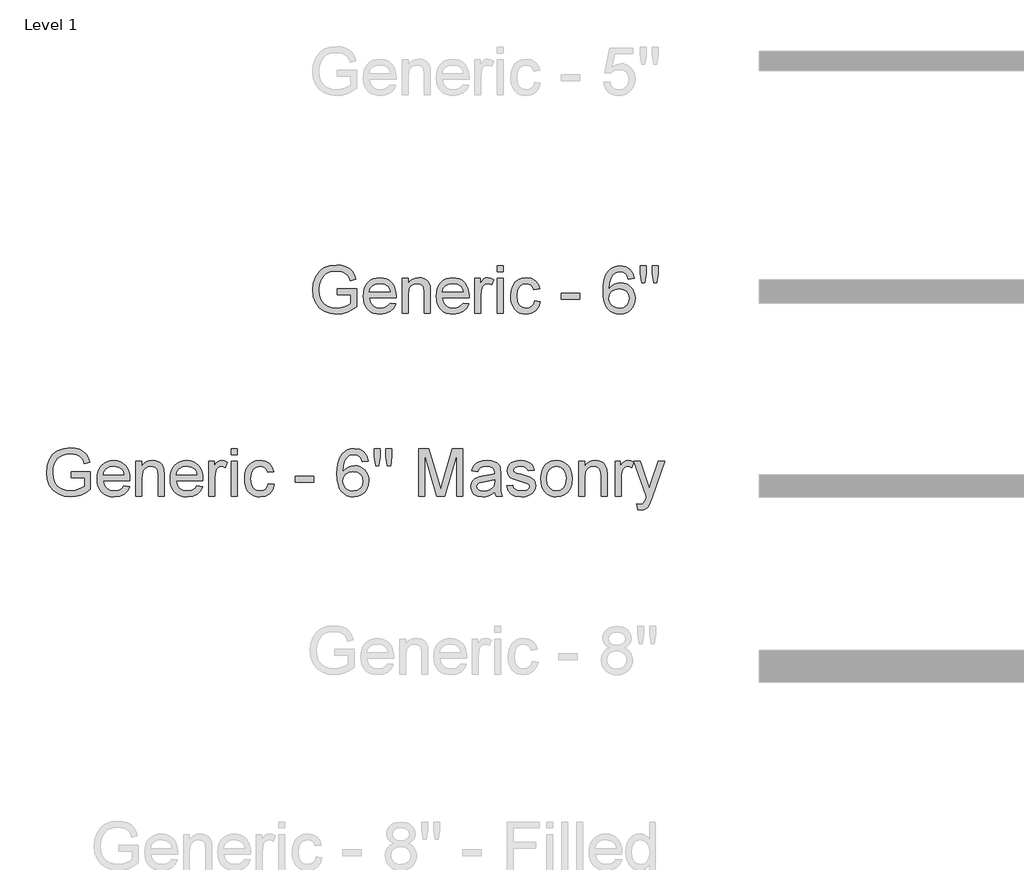
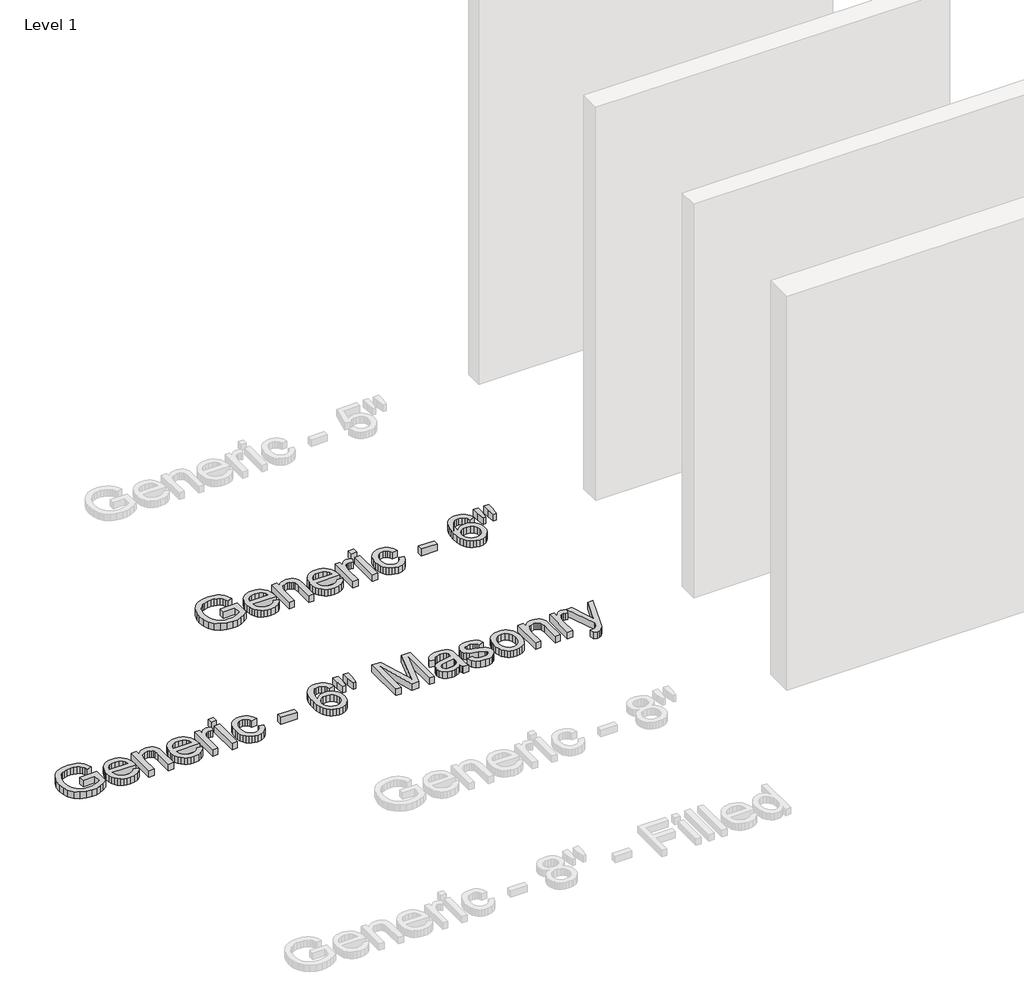
# One storey, part 24 of 42: 2 proxies.
"""IFC4 building model written with IfcOpenShell, lengths in millimetres."""

from ifc_helpers import new_model, si_unit, origin, origin_with_axes, place, context, project, spatial, polyline, outline, extrude, element, save

model = new_model("IFC4")

# Units and contexts
model_context = context("Model", 3, world=origin())
ifc_project = project(units=[si_unit("LENGTHUNIT", "METRE", prefix="MILLI")], contexts=[model_context])

# Site, building, storey
site = spatial("IfcSite", under=ifc_project)
building = spatial("IfcBuilding", under=site)
storey = spatial("IfcBuildingStorey", under=building, Name="Level 1", Elevation=0.0)

# Proxies
placement = place(None, origin())
element("IfcBuildingElementProxy", 1, Name="8\" Arial", ObjectType="8\" Arial", at=placement, inside=storey, context=model_context, shape_type="SweptSolid", body=[
    extrude(outline(polyline([(-15218.2716605, 14606.7864432), (-15218.2716605, 14644.85733), (-15094.5412786, 14644.85733), (-15094.5412786, 14531.0164557), (-15124.6094716, 14510.103493), (-15155.6257189, 14495.1019278), (-15187.5156634, 14486.0675279), (-15220.2049477, 14483.0560613), (-15262.9138649, 14487.8428061), (-15301.5145467, 14502.2030404), (-15333.5810895, 14525.6348533), (-15356.6875896, 14557.6363336), (-15370.6574487, 14596.0232384), (-15375.3140684, 14638.6113251), (-15370.676038, 14681.5061353), (-15356.7619468, 14721.4080681), (-15334.1480632, 14754.8781031), (-15319.7947998, 14767.9115262), (-15303.4106553, 14778.4772196), (-15265.9718048, 14792.4749627), (-15223.253593, 14797.140877), (-15191.8934436, 14794.4361338), (-15163.6934752, 14786.3219043), (-15139.9456442, 14773.3837514), (-15121.941907, 14756.207238), (-15108.6226734, 14733.9651404), (-15098.9283534, 14705.8302346), (-15134.0249521, 14695.9407269), (-15141.8603421, 14716.0078764), (-15151.3873585, 14731.1488614), (-15163.990904, 14742.5626917), (-15181.0558816, 14751.4483772), (-15201.4018706, 14757.164587), (-15223.8484506, 14759.0699903), (-15250.1244264, 14757.0158726), (-15272.5895956, 14750.8535196), (-15291.1603065, 14741.3543872), (-15305.7529071, 14729.2899314), (-15325.3460295, 14699.9560157), (-15334.2688936, 14671.2169576), (-15337.2431816, 14640.1728263), (-15333.6647414, 14603.7656819), (-15322.9294205, 14573.8090247), (-15305.3625318, 14550.5166316), (-15281.2893881, 14534.1022795), (-15253.1173037, 14524.3707809), (-15223.253593, 14521.126948), (-15196.8846707, 14523.571441), (-15171.1663739, 14530.9049199), (-15148.8313297, 14541.0082046), (-15132.6121653, 14551.7621147), (-15132.6121653, 14606.7864432), (-15218.2716605, 14606.7864432)])), origin_with_axes(), (0.0, 0.0, 1.0), 50.8),
    extrude(outline(polyline([(-14880.8386837, 14554.4389739), (-14843.511369, 14549.6801131), (-14856.9607277, 14521.5545019), (-14878.4220747, 14500.5300034), (-14907.4120883, 14487.4245468), (-14943.4474467, 14483.0560613), (-14967.0697999, 14484.9405516), (-14988.117535, 14490.5940225), (-15006.5906521, 14500.016474), (-15022.4891511, 14513.2079061), (-15035.2739423, 14529.8011802), (-15044.405936, 14549.4291575), (-15049.8851322, 14572.0918381), (-15051.7115309, 14597.7892219), (-15049.8665429, 14624.3579792), (-15044.3315788, 14647.7758501), (-15035.1066386, 14668.0428346), (-15022.1917223, 14685.1589328), (-15006.3350492, 14698.7570058), (-14988.2848387, 14708.4699152), (-14968.0410909, 14714.2976608), (-14945.6038055, 14716.2402427), (-14923.8891793, 14714.3023081), (-14904.2519073, 14708.4885045), (-14886.6919896, 14698.7988318), (-14871.2094262, 14685.23329), (-14858.5710258, 14668.1543704), (-14849.5435969, 14647.9245645), (-14844.1271396, 14624.5438722), (-14842.3216538, 14598.0122935), (-14842.5447254, 14587.7509998), (-15013.6406442, 14587.7509998), (-15007.0507373, 14559.2536027), (-14991.7424486, 14538.3034614), (-14969.6490653, 14525.4210764), (-14942.7038747, 14521.126948), (-14922.4415375, 14523.1160031), (-14905.37656, 14529.0831685), (-14891.508942, 14539.4002301), (-14880.8386837, 14554.4389739)]), holes=[polyline([(-15013.6406442, 14625.8218866), (-14880.3925405, 14625.8218866), (-14885.5417767, 14645.9355094), (-14895.6357667, 14660.3236277), (-14917.8313911, 14673.7079239), (-14945.7525199, 14678.1693559), (-14971.4150488, 14674.6095049), (-14992.634735, 14663.929952), (-15007.3853447, 14647.2832337), (-15013.6406442, 14625.8218866)])]), origin_with_axes(), (0.0, 0.0, 1.0), 50.8),
    extrude(outline(polyline([(-14804.250767, 14487.8149221), (-14804.250767, 14711.4813818), (-14766.1798803, 14711.4813818), (-14766.1798803, 14680.2513575), (-14752.9535932, 14695.9964948), (-14737.0690362, 14707.2430214), (-14718.5262093, 14713.9909373), (-14697.3251124, 14716.2402427), (-14678.5592139, 14714.4277859), (-14661.3734059, 14708.9904156), (-14647.0410554, 14700.6066412), (-14636.8355296, 14689.9549722), (-14625.4216993, 14661.9594861), (-14623.4140549, 14625.1526718), (-14623.4140549, 14487.8149221), (-14661.4849417, 14487.8149221), (-14661.4849417, 14620.0220249), (-14665.8720165, 14653.7058369), (-14671.941423, 14663.7347643), (-14681.3754929, 14671.5143864), (-14693.4678326, 14676.5056135), (-14707.5120489, 14678.1693559), (-14729.8099145, 14674.4329066), (-14748.8174739, 14663.2235586), (-14756.4135267, 14654.0729755), (-14761.8392787, 14641.5670238), (-14766.1798803, 14606.4890144), (-14766.1798803, 14487.8149221), (-14804.250767, 14487.8149221)])), origin_with_axes(), (0.0, 0.0, 1.0), 50.8),
    extrude(outline(polyline([(-14414.4703209, 14554.4389739), (-14377.1430062, 14549.6801131), (-14390.5923649, 14521.5545019), (-14412.0537119, 14500.5300034), (-14441.0437255, 14487.4245468), (-14477.0790839, 14483.0560613), (-14500.7014371, 14484.9405516), (-14521.7491723, 14490.5940225), (-14540.2222893, 14500.016474), (-14556.1207883, 14513.2079061), (-14568.9055795, 14529.8011802), (-14578.0375732, 14549.4291575), (-14583.5167694, 14572.0918381), (-14585.3431682, 14597.7892219), (-14583.4981801, 14624.3579792), (-14577.963216, 14647.7758501), (-14568.7382758, 14668.0428346), (-14555.8233595, 14685.1589328), (-14539.9666864, 14698.7570058), (-14521.916476, 14708.4699152), (-14501.6727281, 14714.2976608), (-14479.2354428, 14716.2402427), (-14457.5208165, 14714.3023081), (-14437.8835445, 14708.4885045), (-14420.3236268, 14698.7988318), (-14404.8410635, 14685.23329), (-14392.202663, 14668.1543704), (-14383.1752341, 14647.9245645), (-14377.7587768, 14624.5438722), (-14375.953291, 14598.0122935), (-14376.1763626, 14587.7509998), (-14547.2722814, 14587.7509998), (-14540.6823745, 14559.2536027), (-14525.3740858, 14538.3034614), (-14503.2807025, 14525.4210764), (-14476.3355119, 14521.126948), (-14456.0731747, 14523.1160031), (-14439.0081972, 14529.0831685), (-14425.1405792, 14539.4002301), (-14414.4703209, 14554.4389739)]), holes=[polyline([(-14547.2722814, 14625.8218866), (-14414.0241777, 14625.8218866), (-14419.1734139, 14645.9355094), (-14429.2674039, 14660.3236277), (-14451.4630283, 14673.7079239), (-14479.3841572, 14678.1693559), (-14505.046686, 14674.6095049), (-14526.2663722, 14663.929952), (-14541.0169819, 14647.2832337), (-14547.2722814, 14625.8218866)])]), origin_with_axes(), (0.0, 0.0, 1.0), 50.8),
    extrude(outline(polyline([(-14337.8824042, 14487.8149221), (-14337.8824042, 14711.4813818), (-14304.5703783, 14711.4813818), (-14304.5703783, 14678.3924275), (-14292.2642616, 14697.5765853), (-14280.9247885, 14708.8788798), (-14269.5481368, 14714.3999019), (-14257.1304843, 14716.2402427), (-14238.1693981, 14713.3031332), (-14218.9108831, 14704.4918049), (-14231.6259644, 14670.3618498), (-14245.0102605, 14676.2174794), (-14258.3945567, 14678.1693559), (-14269.7619137, 14676.2918366), (-14279.9209663, 14670.6592786), (-14288.1281423, 14661.6992359), (-14293.6398698, 14649.8392624), (-14298.2686056, 14628.573103), (-14299.8115175, 14605.3736564), (-14299.8115175, 14487.8149221), (-14337.8824042, 14487.8149221)])), origin_with_axes(), (0.0, 0.0, 1.0), 50.8),
    extrude(outline(polyline([(-14195.1165789, 14754.3111294), (-14195.1165789, 14792.3820162), (-14157.0456921, 14792.3820162), (-14157.0456921, 14754.3111294), (-14195.1165789, 14754.3111294)])), origin_with_axes(), (0.0, 0.0, 1.0), 50.8),
    extrude(outline(polyline([(-14195.1165789, 14487.8149221), (-14195.1165789, 14711.4813818), (-14157.0456921, 14711.4813818), (-14157.0456921, 14487.8149221), (-14195.1165789, 14487.8149221)])), origin_with_axes(), (0.0, 0.0, 1.0), 50.8),
    extrude(outline(polyline([(-13957.1735366, 14568.7155565), (-13919.1026499, 14563.9566956), (-13929.7171403, 14530.0962853), (-13949.6634594, 14504.5081137), (-13977.0640878, 14488.4190744), (-14010.0415063, 14483.0560613), (-14031.3936413, 14484.9266096), (-14050.5382968, 14490.5382546), (-14067.4754729, 14499.8909962), (-14082.2051696, 14512.9848345), (-14094.127882, 14529.5734613), (-14102.6441052, 14549.4105682), (-14107.753839, 14572.4961554), (-14109.4570837, 14598.8302227), (-14106.5478582, 14632.7092223), (-14097.8201818, 14662.0710219), (-14083.1346346, 14685.7816743), (-14062.351797, 14702.7072321), (-14037.488608, 14712.85699), (-14010.5620067, 14716.2402427), (-13978.3932228, 14711.5929176), (-13952.674926, 14697.6509425), (-13934.2250456, 14675.1578893), (-13923.8615107, 14644.85733), (-13961.9323975, 14640.0984691), (-13968.8383225, 14656.7080088), (-13979.5922327, 14668.6144556), (-13993.5992703, 14675.7806308), (-14010.2645779, 14678.1693559), (-14034.8675167, 14673.4662629), (-14054.3955766, 14659.3569841), (-14067.1385418, 14635.0793581), (-14071.3861969, 14599.8712236), (-14067.2314883, 14564.1890619), (-14054.7673626, 14539.827784), (-14035.5924994, 14525.802157), (-14011.3055787, 14521.126948), (-13991.5916259, 14524.0454681), (-13975.4282294, 14532.8010285), (-13963.6704971, 14547.6167008), (-13957.1735366, 14568.7155565)])), origin_with_axes(), (0.0, 0.0, 1.0), 50.8),
    extrude(outline(polyline([(-13785.8545462, 14578.2332782), (-13785.8545462, 14616.3041649), (-13666.8830251, 14616.3041649), (-13666.8830251, 14578.2332782), (-13785.8545462, 14578.2332782)])), origin_with_axes(), (0.0, 0.0, 1.0), 50.8),
    extrude(outline(polyline([(-13319.4861834, 14711.4813818), (-13357.5570702, 14706.722521), (-13363.6915392, 14725.5906606), (-13371.9823671, 14738.4730457), (-13389.251827, 14750.3516085), (-13410.1276111, 14754.3111294), (-13427.8246249, 14752.0060562), (-13444.4806378, 14745.0908365), (-13458.7851043, 14730.5261198), (-13470.4684795, 14710.4775596), (-13478.3596374, 14682.1195822), (-13481.2874522, 14642.626614), (-13466.0163421, 14660.4444582), (-13447.715176, 14673.0015304), (-13427.4063656, 14680.4465452), (-13406.1123222, 14682.9282167), (-13387.8204509, 14681.2319431), (-13370.9413663, 14676.1431222), (-13355.4750686, 14667.661754), (-13341.4215576, 14655.7878385), (-13329.7428298, 14641.2277691), (-13321.4008814, 14624.6879393), (-13316.3957123, 14606.168349), (-13314.7273226, 14585.6689982), (-13317.8689143, 14558.4077895), (-13327.2936895, 14533.1356359), (-13342.2208975, 14511.7021728), (-13361.8697878, 14495.9570356), (-13385.348074, 14486.2813048), (-13411.7634695, 14483.0560613), (-13434.4586814, 14485.1938308), (-13454.9557085, 14491.6071393), (-13473.2545508, 14502.2959869), (-13489.3552084, 14517.2603736), (-13502.481578, 14537.1323355), (-13511.8575563, 14562.5439088), (-13517.4831433, 14593.4950936), (-13519.3583389, 14629.9858898), (-13517.2763373, 14670.8962922), (-13511.0303324, 14705.8116453), (-13500.6203243, 14734.731949), (-13486.046313, 14757.6572034), (-13470.2500552, 14772.849309), (-13451.9349472, 14783.700813), (-13431.100989, 14790.2117154), (-13407.7481807, 14792.3820162), (-13374.3432082, 14787.0097084), (-13347.5932053, 14770.8927852), (-13328.8551907, 14745.2953188), (-13319.4861834, 14711.4813818)]), holes=[polyline([(-13481.2874522, 14586.2638558), (-13479.0846201, 14569.3940659), (-13472.4761239, 14553.2864373), (-13462.2148302, 14539.4374087), (-13449.0536057, 14529.3434187), (-13433.1690487, 14523.1810657), (-13414.7377575, 14521.126948), (-13389.6143183, 14525.3838978), (-13369.8631869, 14538.154747), (-13357.0644537, 14558.2311912), (-13352.7982093, 14584.4049258), (-13357.0086858, 14609.528365), (-13369.6401153, 14628.6846388), (-13389.7258541, 14640.8141572), (-13416.2992587, 14644.85733), (-13441.3855193, 14640.8141572), (-13462.3635446, 14628.6846388), (-13476.5564753, 14609.9930975), (-13481.2874522, 14586.2638558)])]), origin_with_axes(), (0.0, 0.0, 1.0), 50.8),
    extrude(outline(polyline([(-13272.1206466, 14682.9282167), (-13281.4152967, 14741.7447625), (-13281.4152967, 14792.3820162), (-13243.3444099, 14792.3820162), (-13243.3444099, 14741.7447625), (-13251.6724164, 14682.9282167), (-13272.1206466, 14682.9282167)])), origin_with_axes(), (0.0, 0.0, 1.0), 50.8),
    extrude(outline(polyline([(-13196.2019447, 14682.9282167), (-13205.2735232, 14741.7447625), (-13205.2735232, 14792.3820162), (-13167.2026364, 14792.3820162), (-13167.2026364, 14741.7447625), (-13176.1255005, 14682.9282167), (-13196.2019447, 14682.9282167)])), origin_with_axes(), (0.0, 0.0, 1.0), 50.8),
])
element("IfcBuildingElementProxy", 2, Name="8\" Arial", ObjectType="8\" Arial", at=placement, inside=storey, context=model_context, shape_type="SweptSolid", body=[
    extrude(outline(polyline([(-16920.0716605, 13438.3864432), (-16920.0716605, 13476.45733), (-16796.3412786, 13476.45733), (-16796.3412786, 13362.6164557), (-16826.4094716, 13341.703493), (-16857.4257189, 13326.7019278), (-16889.3156634, 13317.6675279), (-16922.0049477, 13314.6560613), (-16964.7138649, 13319.4428061), (-17003.3145467, 13333.8030404), (-17035.3810895, 13357.2348533), (-17058.4875896, 13389.2363336), (-17072.4574487, 13427.6232384), (-17077.1140684, 13470.2113251), (-17072.476038, 13513.1061353), (-17058.5619468, 13553.0080681), (-17035.9480632, 13586.4781031), (-17021.5947998, 13599.5115262), (-17005.2106553, 13610.0772196), (-16967.7718048, 13624.0749627), (-16925.053593, 13628.740877), (-16893.6934436, 13626.0361338), (-16865.4934752, 13617.9219043), (-16841.7456442, 13604.9837514), (-16823.741907, 13587.807238), (-16810.4226734, 13565.5651404), (-16800.7283534, 13537.4302346), (-16835.8249521, 13527.5407269), (-16843.6603421, 13547.6078764), (-16853.1873585, 13562.7488614), (-16865.790904, 13574.1626917), (-16882.8558816, 13583.0483772), (-16903.2018706, 13588.764587), (-16925.6484506, 13590.6699903), (-16951.9244264, 13588.6158726), (-16974.3895956, 13582.4535196), (-16992.9603065, 13572.9543872), (-17007.5529071, 13560.8899314), (-17027.1460295, 13531.5560157), (-17036.0688936, 13502.8169576), (-17039.0431816, 13471.7728263), (-17035.4647414, 13435.3656819), (-17024.7294205, 13405.4090247), (-17007.1625318, 13382.1166316), (-16983.0893881, 13365.7022795), (-16954.9173037, 13355.9707809), (-16925.053593, 13352.726948), (-16898.6846707, 13355.171441), (-16872.9663739, 13362.5049199), (-16850.6313297, 13372.6082046), (-16834.4121653, 13383.3621147), (-16834.4121653, 13438.3864432), (-16920.0716605, 13438.3864432)])), origin_with_axes(), (0.0, 0.0, 1.0), 50.8),
    extrude(outline(polyline([(-16582.6386837, 13386.0389739), (-16545.311369, 13381.2801131), (-16558.7607277, 13353.1545019), (-16580.2220747, 13332.1300034), (-16609.2120883, 13319.0245468), (-16645.2474467, 13314.6560613), (-16668.8697999, 13316.5405516), (-16689.917535, 13322.1940225), (-16708.3906521, 13331.616474), (-16724.2891511, 13344.8079061), (-16737.0739423, 13361.4011802), (-16746.205936, 13381.0291575), (-16751.6851322, 13403.6918381), (-16753.5115309, 13429.3892219), (-16751.6665429, 13455.9579792), (-16746.1315788, 13479.3758501), (-16736.9066386, 13499.6428346), (-16723.9917223, 13516.7589328), (-16708.1350492, 13530.3570058), (-16690.0848387, 13540.0699152), (-16669.8410909, 13545.8976608), (-16647.4038055, 13547.8402427), (-16625.6891793, 13545.9023081), (-16606.0519073, 13540.0885045), (-16588.4919896, 13530.3988318), (-16573.0094262, 13516.83329), (-16560.3710258, 13499.7543704), (-16551.3435969, 13479.5245645), (-16545.9271396, 13456.1438722), (-16544.1216538, 13429.6122935), (-16544.3447254, 13419.3509998), (-16715.4406442, 13419.3509998), (-16708.8507373, 13390.8536027), (-16693.5424486, 13369.9034614), (-16671.4490653, 13357.0210764), (-16644.5038747, 13352.726948), (-16624.2415375, 13354.7160031), (-16607.17656, 13360.6831685), (-16593.308942, 13371.0002301), (-16582.6386837, 13386.0389739)]), holes=[polyline([(-16715.4406442, 13457.4218866), (-16582.1925405, 13457.4218866), (-16587.3417767, 13477.5355094), (-16597.4357667, 13491.9236277), (-16619.6313911, 13505.3079239), (-16647.5525199, 13509.7693559), (-16673.2150488, 13506.2095049), (-16694.434735, 13495.529952), (-16709.1853447, 13478.8832337), (-16715.4406442, 13457.4218866)])]), origin_with_axes(), (0.0, 0.0, 1.0), 50.8),
    extrude(outline(polyline([(-16506.050767, 13319.4149221), (-16506.050767, 13543.0813818), (-16467.9798803, 13543.0813818), (-16467.9798803, 13511.8513575), (-16454.7535932, 13527.5964948), (-16438.8690362, 13538.8430214), (-16420.3262093, 13545.5909373), (-16399.1251124, 13547.8402427), (-16380.3592139, 13546.0277859), (-16363.1734059, 13540.5904156), (-16348.8410554, 13532.2066412), (-16338.6355296, 13521.5549722), (-16327.2216993, 13493.5594861), (-16325.2140549, 13456.7526718), (-16325.2140549, 13319.4149221), (-16363.2849417, 13319.4149221), (-16363.2849417, 13451.6220249), (-16367.6720165, 13485.3058369), (-16373.741423, 13495.3347643), (-16383.1754929, 13503.1143864), (-16395.2678326, 13508.1056135), (-16409.3120489, 13509.7693559), (-16431.6099145, 13506.0329066), (-16450.6174739, 13494.8235586), (-16458.2135267, 13485.6729755), (-16463.6392787, 13473.1670238), (-16467.9798803, 13438.0890144), (-16467.9798803, 13319.4149221), (-16506.050767, 13319.4149221)])), origin_with_axes(), (0.0, 0.0, 1.0), 50.8),
    extrude(outline(polyline([(-16116.2703209, 13386.0389739), (-16078.9430062, 13381.2801131), (-16092.3923649, 13353.1545019), (-16113.8537119, 13332.1300034), (-16142.8437255, 13319.0245468), (-16178.8790839, 13314.6560613), (-16202.5014371, 13316.5405516), (-16223.5491723, 13322.1940225), (-16242.0222893, 13331.616474), (-16257.9207883, 13344.8079061), (-16270.7055795, 13361.4011802), (-16279.8375732, 13381.0291575), (-16285.3167694, 13403.6918381), (-16287.1431682, 13429.3892219), (-16285.2981801, 13455.9579792), (-16279.763216, 13479.3758501), (-16270.5382758, 13499.6428346), (-16257.6233595, 13516.7589328), (-16241.7666864, 13530.3570058), (-16223.716476, 13540.0699152), (-16203.4727281, 13545.8976608), (-16181.0354428, 13547.8402427), (-16159.3208165, 13545.9023081), (-16139.6835445, 13540.0885045), (-16122.1236268, 13530.3988318), (-16106.6410635, 13516.83329), (-16094.002663, 13499.7543704), (-16084.9752341, 13479.5245645), (-16079.5587768, 13456.1438722), (-16077.753291, 13429.6122935), (-16077.9763626, 13419.3509998), (-16249.0722814, 13419.3509998), (-16242.4823745, 13390.8536027), (-16227.1740858, 13369.9034614), (-16205.0807025, 13357.0210764), (-16178.1355119, 13352.726948), (-16157.8731747, 13354.7160031), (-16140.8081972, 13360.6831685), (-16126.9405792, 13371.0002301), (-16116.2703209, 13386.0389739)]), holes=[polyline([(-16249.0722814, 13457.4218866), (-16115.8241777, 13457.4218866), (-16120.9734139, 13477.5355094), (-16131.0674039, 13491.9236277), (-16153.2630283, 13505.3079239), (-16181.1841572, 13509.7693559), (-16206.846686, 13506.2095049), (-16228.0663722, 13495.529952), (-16242.8169819, 13478.8832337), (-16249.0722814, 13457.4218866)])]), origin_with_axes(), (0.0, 0.0, 1.0), 50.8),
    extrude(outline(polyline([(-16039.6824042, 13319.4149221), (-16039.6824042, 13543.0813818), (-16006.3703783, 13543.0813818), (-16006.3703783, 13509.9924275), (-15994.0642616, 13529.1765853), (-15982.7247885, 13540.4788798), (-15971.3481368, 13545.9999019), (-15958.9304843, 13547.8402427), (-15939.9693981, 13544.9031332), (-15920.7108831, 13536.0918049), (-15933.4259644, 13501.9618498), (-15946.8102605, 13507.8174794), (-15960.1945567, 13509.7693559), (-15971.5619137, 13507.8918366), (-15981.7209663, 13502.2592786), (-15989.9281423, 13493.2992359), (-15995.4398698, 13481.4392624), (-16000.0686056, 13460.173103), (-16001.6115175, 13436.9736564), (-16001.6115175, 13319.4149221), (-16039.6824042, 13319.4149221)])), origin_with_axes(), (0.0, 0.0, 1.0), 50.8),
    extrude(outline(polyline([(-15896.9165789, 13585.9111294), (-15896.9165789, 13623.9820162), (-15858.8456921, 13623.9820162), (-15858.8456921, 13585.9111294), (-15896.9165789, 13585.9111294)])), origin_with_axes(), (0.0, 0.0, 1.0), 50.8),
    extrude(outline(polyline([(-15896.9165789, 13319.4149221), (-15896.9165789, 13543.0813818), (-15858.8456921, 13543.0813818), (-15858.8456921, 13319.4149221), (-15896.9165789, 13319.4149221)])), origin_with_axes(), (0.0, 0.0, 1.0), 50.8),
    extrude(outline(polyline([(-15658.9735366, 13400.3155565), (-15620.9026499, 13395.5566956), (-15631.5171403, 13361.6962853), (-15651.4634594, 13336.1081137), (-15678.8640878, 13320.0190744), (-15711.8415063, 13314.6560613), (-15733.1936413, 13316.5266096), (-15752.3382968, 13322.1382546), (-15769.2754729, 13331.4909962), (-15784.0051696, 13344.5848345), (-15795.927882, 13361.1734613), (-15804.4441052, 13381.0105682), (-15809.553839, 13404.0961554), (-15811.2570837, 13430.4302227), (-15808.3478582, 13464.3092223), (-15799.6201818, 13493.6710219), (-15784.9346346, 13517.3816743), (-15764.151797, 13534.3072321), (-15739.288608, 13544.45699), (-15712.3620067, 13547.8402427), (-15680.1932228, 13543.1929176), (-15654.474926, 13529.2509425), (-15636.0250456, 13506.7578893), (-15625.6615107, 13476.45733), (-15663.7323975, 13471.6984691), (-15670.6383225, 13488.3080088), (-15681.3922327, 13500.2144556), (-15695.3992703, 13507.3806308), (-15712.0645779, 13509.7693559), (-15736.6675167, 13505.0662629), (-15756.1955766, 13490.9569841), (-15768.9385418, 13466.6793581), (-15773.1861969, 13431.4712236), (-15769.0314883, 13395.7890619), (-15756.5673626, 13371.427784), (-15737.3924994, 13357.402157), (-15713.1055787, 13352.726948), (-15693.3916259, 13355.6454681), (-15677.2282294, 13364.4010285), (-15665.4704971, 13379.2167008), (-15658.9735366, 13400.3155565)])), origin_with_axes(), (0.0, 0.0, 1.0), 50.8),
    extrude(outline(polyline([(-15487.6545462, 13409.8332782), (-15487.6545462, 13447.9041649), (-15368.6830251, 13447.9041649), (-15368.6830251, 13409.8332782), (-15487.6545462, 13409.8332782)])), origin_with_axes(), (0.0, 0.0, 1.0), 50.8),
    extrude(outline(polyline([(-15021.2861834, 13543.0813818), (-15059.3570702, 13538.322521), (-15065.4915392, 13557.1906606), (-15073.7823671, 13570.0730457), (-15091.051827, 13581.9516085), (-15111.9276111, 13585.9111294), (-15129.6246249, 13583.6060562), (-15146.2806378, 13576.6908365), (-15160.5851043, 13562.1261198), (-15172.2684795, 13542.0775596), (-15180.1596374, 13513.7195822), (-15183.0874522, 13474.226614), (-15167.8163421, 13492.0444582), (-15149.515176, 13504.6015304), (-15129.2063656, 13512.0465452), (-15107.9123222, 13514.5282167), (-15089.6204509, 13512.8319431), (-15072.7413663, 13507.7431222), (-15057.2750686, 13499.261754), (-15043.2215576, 13487.3878385), (-15031.5428298, 13472.8277691), (-15023.2008814, 13456.2879393), (-15018.1957123, 13437.768349), (-15016.5273226, 13417.2689982), (-15019.6689143, 13390.0077895), (-15029.0936895, 13364.7356359), (-15044.0208975, 13343.3021728), (-15063.6697878, 13327.5570356), (-15087.148074, 13317.8813048), (-15113.5634695, 13314.6560613), (-15136.2586814, 13316.7938308), (-15156.7557085, 13323.2071393), (-15175.0545508, 13333.8959869), (-15191.1552084, 13348.8603736), (-15204.281578, 13368.7323355), (-15213.6575563, 13394.1439088), (-15219.2831433, 13425.0950936), (-15221.1583389, 13461.5858898), (-15219.0763373, 13502.4962922), (-15212.8303324, 13537.4116453), (-15202.4203243, 13566.331949), (-15187.846313, 13589.2572034), (-15172.0500552, 13604.449309), (-15153.7349472, 13615.300813), (-15132.900989, 13621.8117154), (-15109.5481807, 13623.9820162), (-15076.1432082, 13618.6097084), (-15049.3932053, 13602.4927852), (-15030.6551907, 13576.8953188), (-15021.2861834, 13543.0813818)]), holes=[polyline([(-15183.0874522, 13417.8638558), (-15180.8846201, 13400.9940659), (-15174.2761239, 13384.8864373), (-15164.0148302, 13371.0374087), (-15150.8536057, 13360.9434187), (-15134.9690487, 13354.7810657), (-15116.5377575, 13352.726948), (-15091.4143183, 13356.9838978), (-15071.6631869, 13369.754747), (-15058.8644537, 13389.8311912), (-15054.5982093, 13416.0049258), (-15058.8086858, 13441.128365), (-15071.4401153, 13460.2846388), (-15091.5258541, 13472.4141572), (-15118.0992587, 13476.45733), (-15143.1855193, 13472.4141572), (-15164.1635446, 13460.2846388), (-15178.3564753, 13441.5930975), (-15183.0874522, 13417.8638558)])]), origin_with_axes(), (0.0, 0.0, 1.0), 50.8),
    extrude(outline(polyline([(-14973.9206466, 13514.5282167), (-14983.2152967, 13573.3447625), (-14983.2152967, 13623.9820162), (-14945.1444099, 13623.9820162), (-14945.1444099, 13573.3447625), (-14953.4724164, 13514.5282167), (-14973.9206466, 13514.5282167)])), origin_with_axes(), (0.0, 0.0, 1.0), 50.8),
    extrude(outline(polyline([(-14898.0019447, 13514.5282167), (-14907.0735232, 13573.3447625), (-14907.0735232, 13623.9820162), (-14869.0026364, 13623.9820162), (-14869.0026364, 13573.3447625), (-14877.9255005, 13514.5282167), (-14898.0019447, 13514.5282167)])), origin_with_axes(), (0.0, 0.0, 1.0), 50.8),
    extrude(outline(polyline([(-14697.683646, 13319.4149221), (-14697.683646, 13623.9820162), (-14632.1749522, 13623.9820162), (-14569.863618, 13409.3127777), (-14557.2972511, 13364.4753857), (-14543.6898833, 13413.0306378), (-14482.41955, 13623.9820162), (-14416.9108561, 13623.9820162), (-14416.9108561, 13319.4149221), (-14454.9817429, 13319.4149221), (-14454.9817429, 13585.9111294), (-14531.4953024, 13319.4149221), (-14583.0991997, 13319.4149221), (-14659.6127592, 13585.9111294), (-14659.6127592, 13319.4149221), (-14697.683646, 13319.4149221)])), origin_with_axes(), (0.0, 0.0, 1.0), 50.8),
    extrude(outline(polyline([(-14212.2798398, 13347.9680872), (-14230.46947, 13332.3716643), (-14249.19819, 13322.1661385), (-14268.8935535, 13316.5335806), (-14289.9831145, 13314.6560613), (-14321.7987018, 13319.1732612), (-14345.2676933, 13332.724861), (-14359.7394635, 13353.3032163), (-14364.5633868, 13378.9006827), (-14362.7416354, 13394.6829985), (-14357.2763812, 13409.0153489), (-14348.8461336, 13421.2842871), (-14338.129402, 13430.876366), (-14311.4723455, 13443.3683757), (-14278.5321056, 13449.0938801), (-14239.6061111, 13455.1168134), (-14212.5029114, 13462.1807474), (-14212.2798398, 13470.6574683), (-14214.9009311, 13487.6480887), (-14222.7642051, 13498.7644902), (-14240.3496831, 13507.0181395), (-14264.8503807, 13509.7693559), (-14287.5293269, 13507.9383098), (-14303.3674107, 13502.4451716), (-14314.1677941, 13492.2861191), (-14321.7336392, 13476.45733), (-14359.804526, 13481.2161908), (-14353.1960298, 13502.036207), (-14343.334406, 13518.3947912), (-14329.2994844, 13530.9053902), (-14310.1710945, 13540.181451), (-14286.7764603, 13545.9255447), (-14259.9428055, 13547.8402427), (-14234.2059194, 13546.1486163), (-14213.8041624, 13541.0737374), (-14198.4215165, 13533.4428297), (-14187.7419636, 13524.083117), (-14180.6594402, 13512.5112777), (-14176.0678831, 13498.2439898), (-14174.2089531, 13464.9319639), (-14174.2089531, 13417.566427), (-14172.2756658, 13351.425697), (-14164.6912314, 13319.4149221), (-14202.7621181, 13319.4149221), (-14208.8594086, 13332.6505038), (-14212.2798398, 13347.9680872)]), holes=[polyline([(-14212.2798398, 13424.1098607), (-14273.6988876, 13412.4357802), (-14306.4532345, 13406.2641325), (-14321.287496, 13396.2259104), (-14326.4925001, 13381.5775419), (-14323.6576318, 13370.2566581), (-14315.153027, 13360.9805973), (-14301.1645786, 13354.7903603), (-14281.8781797, 13352.726948), (-14261.4299495, 13355.0041373), (-14243.3611497, 13361.8357051), (-14228.7127812, 13371.9018111), (-14218.5258447, 13383.8826151), (-14214.0086447, 13396.2259104), (-14212.5029114, 13413.3280666), (-14212.2798398, 13424.1098607)])]), origin_with_axes(), (0.0, 0.0, 1.0), 50.8),
    extrude(outline(polyline([(-14136.1380663, 13386.0389739), (-14098.0671795, 13390.7978348), (-14092.0628356, 13374.5136078), (-14080.444523, 13362.5420985), (-14063.1378845, 13355.1807356), (-14040.068563, 13352.726948), (-14017.278081, 13354.9762533), (-14001.2541042, 13361.7241693), (-13991.7735611, 13371.5021412), (-13988.6133801, 13382.8416143), (-13991.7921504, 13392.545229), (-14001.3284614, 13399.9437705), (-14040.5147062, 13410.7999218), (-14097.8441079, 13429.4264005), (-14112.3530567, 13438.7861132), (-14122.865306, 13451.1758817), (-14129.2507306, 13465.805661), (-14131.3792055, 13481.8854056), (-14129.6689898, 13496.6360153), (-14124.538343, 13510.2526777), (-14116.4519974, 13522.1963031), (-14105.8746856, 13531.9278017), (-14081.6714168, 13543.1929176), (-14048.9170699, 13547.8402427), (-14024.1375327, 13545.972018), (-14002.5925338, 13540.367344), (-13985.2673061, 13531.574605), (-13973.1470824, 13520.1421854), (-13965.1165047, 13505.224272), (-13960.060215, 13485.9750517), (-13998.1311018, 13481.2161908), (-14002.9364359, 13493.1969948), (-14012.4448629, 13502.2221), (-14026.7493294, 13507.8825419), (-14045.9427818, 13509.7693559), (-14067.8037989, 13507.9661938), (-14082.3778102, 13502.5567074), (-14090.5756916, 13494.7492014), (-14093.3083187, 13485.7519801), (-14088.7725295, 13474.6727572), (-14074.5703041, 13466.2703935), (-14041.7787786, 13458.1654586), (-13985.8993423, 13440.2453732), (-13971.1394379, 13431.6757059), (-13959.9486792, 13419.9458574), (-13952.8940398, 13405.0186494), (-13950.5424933, 13386.8569031), (-13953.3030044, 13368.08171), (-13961.5845377, 13350.4218748), (-13975.0710749, 13335.2623005), (-13993.4465982, 13323.9878899), (-14015.6422226, 13316.9890184), (-14040.5890634, 13314.6560613), (-14078.9759683, 13319.1546719), (-14106.9900436, 13332.6505038), (-14125.6908796, 13354.9948426), (-14136.1380663, 13386.0389739)])), origin_with_axes(), (0.0, 0.0, 1.0), 50.8),
    extrude(outline(polyline([(-13917.2304674, 13431.248152), (-13915.1717024, 13460.214929), (-13908.9954075, 13485.1757118), (-13898.7015825, 13506.1305004), (-13884.2902275, 13523.0792948), (-13869.7812787, 13533.9122095), (-13853.7665966, 13541.6500057), (-13836.2461812, 13546.2926834), (-13817.2200325, 13547.8402427), (-13796.216447, 13545.9557523), (-13777.2251532, 13540.3022814), (-13760.2461511, 13530.8798299), (-13745.2794408, 13517.6883978), (-13733.0639469, 13501.1741282), (-13724.3385942, 13481.7831645), (-13719.1033825, 13459.5155065), (-13717.358312, 13434.3711544), (-13720.4441358, 13395.9098923), (-13729.7016073, 13366.6317445), (-13744.8611816, 13344.705665), (-13765.6533138, 13328.3006076), (-13790.3491991, 13318.0671978), (-13817.2200325, 13314.6560613), (-13838.5303415, 13316.5335806), (-13857.6982336, 13322.1661385), (-13874.7237089, 13331.5537351), (-13889.6067674, 13344.6963703), (-13901.6921362, 13361.3709726), (-13910.3245424, 13381.3544703), (-13915.5039862, 13404.6468634), (-13917.2304674, 13431.248152)]), holes=[polyline([(-13879.1595807, 13431.3225092), (-13874.7539165, 13396.8672413), (-13861.5369241, 13372.3200704), (-13841.6463729, 13357.6252286), (-13817.2200325, 13352.726948), (-13792.9052279, 13357.6531126), (-13773.0518553, 13372.4316062), (-13759.8348629, 13397.3040898), (-13755.4291987, 13432.5122244), (-13759.8627468, 13465.96367), (-13773.1633911, 13490.1762335), (-13793.0446476, 13504.8710753), (-13817.2200325, 13509.7693559), (-13841.6463729, 13504.8896646), (-13861.5369241, 13490.2505907), (-13874.7539165, 13465.7591877), (-13879.1595807, 13431.3225092)])]), origin_with_axes(), (0.0, 0.0, 1.0), 50.8),
    extrude(outline(polyline([(-13674.5285644, 13319.4149221), (-13674.5285644, 13543.0813818), (-13636.4576776, 13543.0813818), (-13636.4576776, 13511.8513575), (-13623.2313905, 13527.5964948), (-13607.3468335, 13538.8430214), (-13588.8040066, 13545.5909373), (-13567.6029097, 13547.8402427), (-13548.8370112, 13546.0277859), (-13531.6512032, 13540.5904156), (-13517.3188528, 13532.2066412), (-13507.113327, 13521.5549722), (-13495.6994967, 13493.5594861), (-13493.6918522, 13456.7526718), (-13493.6918522, 13319.4149221), (-13531.762739, 13319.4149221), (-13531.762739, 13451.6220249), (-13536.1498138, 13485.3058369), (-13542.2192204, 13495.3347643), (-13551.6532902, 13503.1143864), (-13563.74563, 13508.1056135), (-13577.7898462, 13509.7693559), (-13600.0877118, 13506.0329066), (-13619.0952712, 13494.8235586), (-13626.691324, 13485.6729755), (-13632.117076, 13473.1670238), (-13636.4576776, 13438.0890144), (-13636.4576776, 13319.4149221), (-13674.5285644, 13319.4149221)])), origin_with_axes(), (0.0, 0.0, 1.0), 50.8),
    extrude(outline(polyline([(-13441.344383, 13319.4149221), (-13441.344383, 13543.0813818), (-13408.032357, 13543.0813818), (-13408.032357, 13509.9924275), (-13395.7262403, 13529.1765853), (-13384.3867672, 13540.4788798), (-13373.0101155, 13545.9999019), (-13360.592463, 13547.8402427), (-13341.6313768, 13544.9031332), (-13322.3728618, 13536.0918049), (-13335.0879432, 13501.9618498), (-13348.4722393, 13507.8174794), (-13361.8565354, 13509.7693559), (-13373.2238925, 13507.8918366), (-13383.382945, 13502.2592786), (-13391.590121, 13493.2992359), (-13397.1018485, 13481.4392624), (-13401.7305843, 13460.173103), (-13403.2734962, 13436.9736564), (-13403.2734962, 13319.4149221), (-13441.344383, 13319.4149221)])), origin_with_axes(), (0.0, 0.0, 1.0), 50.8),
    extrude(outline(polyline([(-13298.5785576, 13233.7554269), (-13303.3374185, 13270.4135268), (-13284.0045463, 13267.0674528), (-13265.9357465, 13271.2686346), (-13254.8565236, 13282.9798938), (-13244.4465155, 13311.0125584), (-13241.4722275, 13320.2328513), (-13322.3728618, 13543.0813818), (-13282.2199735, 13543.0813818), (-13239.3158687, 13418.9048566), (-13224.3700713, 13369.2342466), (-13209.424274, 13413.104995), (-13165.330454, 13543.0813818), (-13125.4749944, 13543.0813818), (-13203.3269835, 13314.0612037), (-13223.5521421, 13264.3905936), (-13233.9063823, 13248.5339205), (-13245.6362307, 13237.5476441), (-13259.2621877, 13231.1343356), (-13275.3047538, 13228.996566), (-13298.5785576, 13233.7554269)])), origin_with_axes(), (0.0, 0.0, 1.0), 50.8),
])

save(model, "model.ifc")

# Revit data of these elements
# Elements 1, 2 (IfcBuildingElementProxy, "8\" Arial")
#   Phase Created = New Construction
